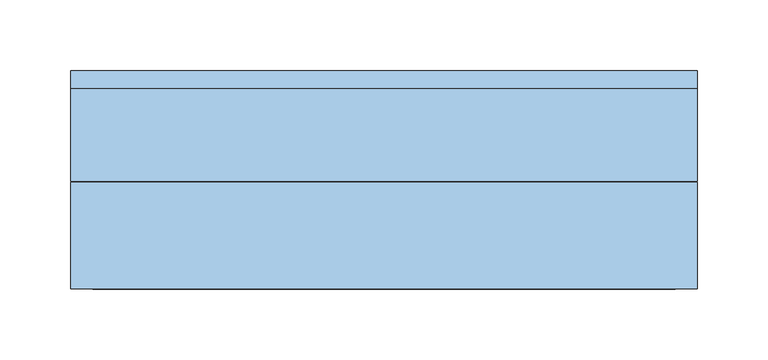
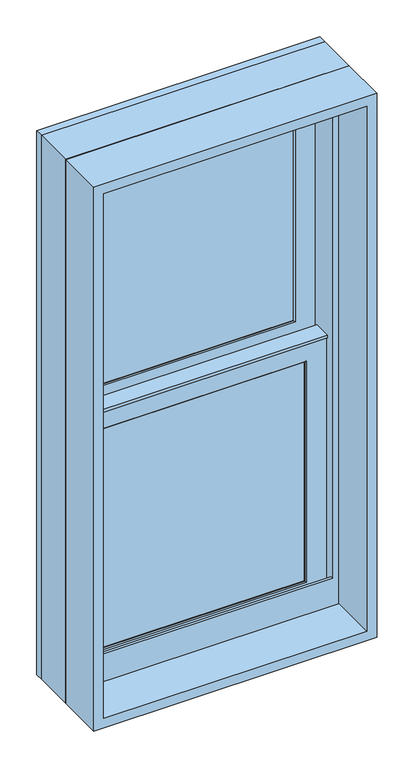
"""IFC4 building model written with IfcOpenShell, lengths in millimetres: window geometry, Window-Double_Hung-Marvin-Essential : ESDH1630."""

from ifc_helpers import new_model, si_unit, frame, origin, place, context, project, spatial, polyline, outline, extrude, faceted_brep, source, transform, mapped, element, save


def window_dba2cc00(model_context):
    return source(origin(), model_context, "Body", "SolidModel", [
        extrude(outline(polyline([(64.5583333, 20.6375), (64.5583333, 15.875), (45.5083333, 15.875), (45.5083333, 20.6375), (64.5583333, 20.6375)])), frame((0.0, 0.0, 1593.85), z_axis=(0.0, 0.0, 1.0), x_axis=(1.0, 0.0, 0.0)), (0.0, 0.0, 1.0), 374.65),
        extrude(outline(polyline([(-45.5083333, 20.6375), (-45.5083333, 15.875), (-64.5583333, 15.875), (-64.5583333, 20.6375), (-45.5083333, 20.6375)])), frame((0.0, 0.0, 1593.85), z_axis=(0.0, 0.0, 1.0), x_axis=(1.0, 0.0, 0.0)), (0.0, 0.0, 1.0), 374.65),
        extrude(outline(polyline([(165.1, 20.6375), (165.1, 15.875), (-165.1, 15.875), (-165.1, 20.6375), (165.1, 20.6375)])), frame((0.0, 0.0, 1771.65), z_axis=(0.0, 0.0, 1.0), x_axis=(1.0, 0.0, 0.0)), (0.0, 0.0, 1.0), 19.05),
        extrude(outline(polyline([(-64.5583333, 46.83125), (-64.5583333, 51.59375), (-45.5083333, 51.59375), (-45.5083333, 46.83125), (-64.5583333, 46.83125)])), frame((0.0, 0.0, 2006.6), z_axis=(0.0, 0.0, 1.0), x_axis=(1.0, 0.0, 0.0)), (0.0, 0.0, 1.0), 374.65),
        extrude(outline(polyline([(45.5083333, 46.83125), (45.5083333, 51.59375), (64.5583333, 51.59375), (64.5583333, 46.83125), (45.5083333, 46.83125)])), frame((0.0, 0.0, 2006.6), z_axis=(0.0, 0.0, 1.0), x_axis=(1.0, 0.0, 0.0)), (0.0, 0.0, 1.0), 374.65),
        extrude(outline(polyline([(-165.1, 46.83125), (-165.1, 51.59375), (165.1, 51.59375), (165.1, 46.83125), (-165.1, 46.83125)])), frame((0.0, 0.0, 2184.4), z_axis=(0.0, 0.0, 1.0), x_axis=(1.0, 0.0, 0.0)), (0.0, 0.0, 1.0), 19.05),
        extrude(outline(polyline([(64.5583333, 20.6375), (45.5083333, 20.6375), (45.5083333, 25.4), (64.5583333, 25.4), (64.5583333, 20.6375)])), frame((0.0, 0.0, 1593.85), z_axis=(0.0, 0.0, 1.0), x_axis=(1.0, 0.0, 0.0)), (0.0, 0.0, 1.0), 374.65),
        extrude(outline(polyline([(-45.5083333, 20.6375), (-64.5583333, 20.6375), (-64.5583333, 25.4), (-45.5083333, 25.4), (-45.5083333, 20.6375)])), frame((0.0, 0.0, 1593.85), z_axis=(0.0, 0.0, 1.0), x_axis=(1.0, 0.0, 0.0)), (0.0, 0.0, 1.0), 374.65),
        extrude(outline(polyline([(165.1, 20.6375), (-165.1, 20.6375), (-165.1, 25.4), (165.1, 25.4), (165.1, 20.6375)])), frame((0.0, 0.0, 1771.65), z_axis=(0.0, 0.0, 1.0), x_axis=(1.0, 0.0, 0.0)), (0.0, 0.0, 1.0), 19.05),
        extrude(outline(polyline([(-64.5583333, 56.35625), (-45.5083333, 56.35625), (-45.5083333, 51.59375), (-64.5583333, 51.59375), (-64.5583333, 56.35625)])), frame((0.0, 0.0, 2006.6), z_axis=(0.0, 0.0, 1.0), x_axis=(1.0, 0.0, 0.0)), (0.0, 0.0, 1.0), 374.65),
        extrude(outline(polyline([(45.5083333, 56.35625), (64.5583333, 56.35625), (64.5583333, 51.59375), (45.5083333, 51.59375), (45.5083333, 56.35625)])), frame((0.0, 0.0, 2006.6), z_axis=(0.0, 0.0, 1.0), x_axis=(1.0, 0.0, 0.0)), (0.0, 0.0, 1.0), 374.65),
        extrude(outline(polyline([(-165.1, 56.35625), (165.1, 56.35625), (165.1, 51.59375), (-165.1, 51.59375), (-165.1, 56.35625)])), frame((0.0, 0.0, 2184.4), z_axis=(0.0, 0.0, 1.0), x_axis=(1.0, 0.0, 0.0)), (0.0, 0.0, 1.0), 19.05),
        faceted_brep([(-192.0875, 5.6780605, 1998.5351748), (-192.0875, 5.6780605, 1993.9), (192.0875, 5.6780605, 1993.9), (192.0875, 5.6780605, 1998.5351748), (-192.0875, 34.8118605, 1998.5351748), (192.0875, 34.8118605, 1998.5351748), (192.0875, 34.8118605, 1993.9), (-192.0875, 34.8118605, 1993.9), (-192.0875, 30.1625, 1993.9), (-192.0875, 30.1625, 1566.8625), (-192.0875, 8.9241104, 1566.8625), (-192.0875, 8.9241104, 1993.9), (192.0875, 8.9241104, 1993.9), (192.0875, 30.1625, 1993.9), (192.0875, 8.9241104, 1566.8625), (192.0875, 30.1625, 1566.8625), (-176.2034752, 11.90625, 1979.6034752), (-176.2034752, 30.1625, 1979.6034752), (176.2034752, 30.1625, 1979.6034752), (176.2034752, 11.90625, 1979.6034752), (-159.54375, 10.4662439, 1962.94375), (-159.54375, 11.90625, 1962.94375), (159.54375, 11.90625, 1962.94375), (159.54375, 10.4662439, 1962.94375), (161.0858834, 8.9241104, 1964.4858834), (-161.0858834, 8.9241104, 1964.4858834), (176.2034752, 30.1625, 1582.7465248), (176.2034752, 11.90625, 1582.7465248), (159.54375, 11.90625, 1599.40625), (159.54375, 10.4662439, 1599.40625), (161.0858834, 8.9241104, 1597.8641166), (-176.2034752, 30.1625, 1582.7465248), (-176.2034752, 11.90625, 1582.7465248), (-159.54375, 11.90625, 1599.40625), (-159.54375, 10.4662439, 1599.40625), (-161.0858834, 8.9241104, 1597.8641166)], [[[0, 1, 2, 3]], [[4, 5, 6, 7]], [[1, 0, 4, 7, 8, 9, 10, 11]], [[2, 1, 11, 12]], [[7, 6, 13, 8]], [[3, 2, 12, 14, 15, 13, 6, 5]], [[0, 3, 5, 4]], [[16, 17, 18, 19]], [[20, 21, 22, 23]], [[20, 23, 24, 25]], [[19, 18, 26, 27]], [[23, 22, 28, 29]], [[24, 23, 29, 30]], [[27, 26, 31, 32]], [[29, 28, 33, 34]], [[30, 29, 34, 35]], [[15, 14, 10, 9]], [[15, 9, 8, 13], [18, 17, 31, 26]], [[17, 16, 32, 31]], [[16, 19, 27, 32], [22, 21, 33, 28]], [[21, 20, 34, 33]], [[20, 25, 35, 34]], [[10, 14, 12, 11], [25, 24, 30, 35]]]),
        extrude(outline(polyline([(38.5955581, 1979.6125), (33.5778968, 1979.6125), (33.5778968, 1981.2), (39.9405976, 1981.2), (39.9405976, 1979.6125), (61.515625, 1979.6125), (47.6307501, 1976.2975159), (38.5955581, 1976.2975159), (38.5955581, 1979.6125)])), frame((-192.0875, 0.0, 0.0), z_axis=(1.0, 0.0, 0.0), x_axis=(0.0, 1.0, 0.0)), (0.0, 0.0, 1.0), 384.175),
        faceted_brep([(222.25, 0.0, 1536.7), (222.25, 0.0, 2438.4), (-222.25, 0.0, 2438.4), (-222.25, 0.0, 1536.7), (196.05625, 0.0, 1597.81875), (-196.05625, 0.0, 1597.81875), (-196.05625, 0.0, 2412.20625), (196.05625, 0.0, 2412.20625), (196.05625, 3.96875, 1536.7), (-196.05625, 3.96875, 1536.7), (-196.05625, 3.96875, 1597.81875), (196.05625, 3.96875, 1597.81875), (-222.25, 65.6828125, 1536.7), (-196.05625, 65.6828125, 1536.7), (196.05625, 65.6828125, 1536.7), (222.25, 65.6828125, 1536.7), (-222.25, 65.6828125, 2438.4), (222.25, 65.6828125, 2438.4), (196.05625, 65.6828125, 2412.20625), (-196.05625, 65.6828125, 2412.20625)], [[[0, 1, 2, 3], [4, 5, 6, 7]], [[8, 9, 10, 11]], [[5, 4, 11, 10]], [[0, 3, 12, 13, 9, 8, 14, 15]], [[13, 12, 16, 17, 15, 14, 18, 19]], [[13, 19, 6, 5, 10, 9]], [[7, 6, 19, 18]], [[18, 14, 8, 11, 4, 7]], [[1, 0, 15, 17]], [[2, 1, 17, 16]], [[3, 2, 16, 12]]]),
        faceted_brep([(196.05625, 30.1625, 1987.55), (194.46875, 30.1625, 1987.55), (194.46875, 30.1625, 1561.0544613), (196.05625, 30.1625, 1561.0544613), (-194.46875, 30.1625, 1987.55), (-196.05625, 30.1625, 1987.55), (-196.05625, 30.1625, 1561.0544613), (-194.46875, 30.1625, 1561.0544613), (194.46875, 63.5, 1987.55), (196.05625, 63.5, 1987.55), (196.05625, 63.5, 1554.5743077), (194.46875, 63.5, 1554.5743077), (-196.05625, 63.5, 1987.55), (-194.46875, 63.5, 1987.55), (-194.46875, 63.5, 1554.5743077), (-196.05625, 63.5, 1554.5743077), (207.3108932, 3.96875, 1566.1460105), (207.3108932, 3.96875, 1536.7), (207.3108932, 65.6828125, 1536.7), (207.3108932, 65.6828125, 1554.150012), (-207.3108932, 3.96875, 1536.7), (-207.3108932, 3.96875, 1566.1460105), (-207.3108932, 65.6828125, 1554.150012), (-207.3108932, 65.6828125, 1536.7), (207.3108932, 78.58125, 1551.6428097), (-207.3108932, 78.58125, 1551.6428097), (-205.2971252, 68.2348864, 1553.6539391), (-187.33135, 68.2348864, 1553.6539391), (-187.33135, 65.6828125, 1554.150012), (187.33135, 65.6828125, 1554.150012), (187.33135, 68.2348864, 1553.6539391), (205.2971252, 68.2348864, 1553.6539391), (-222.25, 65.6828125, 1536.7), (-222.25, 78.5948249, 1536.7), (222.25, 78.5948249, 1536.7), (222.25, 65.6828125, 1536.7), (-222.25, 78.58125, 2438.4), (222.25, 78.58125, 2438.4), (207.3108932, 78.58125, 2423.4608932), (-207.3108932, 78.58125, 2423.4608932), (-222.25, 65.6828125, 2438.4), (-205.2971252, 68.2348864, 2421.4471252), (205.2971252, 68.2348864, 2421.4471252), (187.33135, 68.2348864, 2403.48135), (-187.33135, 68.2348864, 2403.48135), (-187.33135, 65.6828125, 2403.48135), (187.33135, 65.6828125, 2403.48135), (222.25, 65.6828125, 2438.4)], [[[0, 1, 2, 3]], [[4, 5, 6, 7]], [[8, 9, 10, 11]], [[12, 13, 14, 15]], [[1, 8, 11, 2]], [[9, 0, 3, 10]], [[1, 0, 9, 8]], [[5, 4, 13, 12]], [[5, 12, 15, 6]], [[13, 4, 7, 14]], [[16, 17, 18, 19]], [[20, 21, 22, 23]], [[24, 25, 26, 27, 28, 22, 21, 16, 19, 29, 30, 31], [3, 2, 11, 10], [7, 6, 15, 14]], [[17, 16, 21, 20]], [[17, 20, 23, 32, 33, 34, 35, 18]], [[34, 33, 36, 37], [25, 24, 38, 39]], [[33, 32, 40, 36]], [[39, 41, 26, 25]], [[41, 42, 31, 30, 43, 44, 27, 26]], [[44, 45, 28, 27]], [[40, 32, 23, 22, 28, 45, 46, 29, 19, 18, 35, 47]], [[36, 40, 47, 37]], [[39, 38, 42, 41]], [[44, 43, 46, 45]], [[34, 37, 47, 35]], [[42, 38, 24, 31]], [[46, 43, 30, 29]]]),
        extrude(outline(polyline([(172.24375, 11.90625), (-172.24375, 11.90625), (-172.24375, 15.08125), (172.24375, 15.08125), (172.24375, 11.90625)])), frame((0.0, 0.0, 1586.70625), z_axis=(0.0, 0.0, 1.0), x_axis=(1.0, 0.0, 0.0)), (0.0, 0.0, 1.0), 388.9375),
        extrude(outline(polyline([(172.24375, 42.8625), (-172.24375, 42.8625), (-172.24375, 46.0375), (172.24375, 46.0375), (172.24375, 42.8625)])), frame((0.0, 0.0, 1999.45625), z_axis=(0.0, 0.0, 1.0), x_axis=(1.0, 0.0, 0.0)), (0.0, 0.0, 1.0), 388.9375),
        faceted_brep([(-159.54375, 31.194477, 1962.94375), (-161.0858834, 32.7366104, 1964.4858834), (161.0858834, 32.7366104, 1964.4858834), (159.54375, 31.194477, 1962.94375), (-159.54375, 30.1625, 1962.94375), (159.54375, 30.1625, 1962.94375), (-192.0875, 32.7366104, 1995.4875), (-192.0875, 30.1625, 1995.4875), (192.0875, 30.1625, 1995.4875), (192.0875, 32.7366104, 1995.4875), (161.0858834, 32.7366104, 1597.8641166), (159.54375, 31.194477, 1599.40625), (159.54375, 30.1625, 1599.40625), (192.0875, 30.1625, 1566.8625), (192.0875, 32.7366104, 1566.8625), (-161.0858834, 32.7366104, 1597.8641166), (-159.54375, 31.194477, 1599.40625), (-159.54375, 30.1625, 1599.40625), (-192.0875, 30.1625, 1566.8625), (-192.0875, 32.7366104, 1566.8625)], [[[0, 1, 2, 3]], [[4, 0, 3, 5]], [[6, 7, 8, 9]], [[3, 2, 10, 11]], [[5, 3, 11, 12]], [[9, 8, 13, 14]], [[11, 10, 15, 16]], [[12, 11, 16, 17]], [[14, 13, 18, 19]], [[9, 14, 19, 6], [1, 15, 10, 2]], [[16, 15, 1, 0]], [[17, 16, 0, 4]], [[7, 18, 13, 8], [5, 12, 17, 4]], [[19, 18, 7, 6]]]),
        faceted_brep([(-176.2034752, 42.8625, 2392.3534752), (-176.2034752, 61.11875, 2392.3534752), (176.2034752, 61.11875, 2392.3534752), (176.2034752, 42.8625, 2392.3534752), (-159.54375, 41.4224939, 2375.69375), (-159.54375, 42.8625, 2375.69375), (159.54375, 42.8625, 2375.69375), (159.54375, 41.4224939, 2375.69375), (-161.0858834, 39.8803604, 2377.2358834), (161.0858834, 39.8803604, 2377.2358834), (-192.0875, 61.11875, 2408.2375), (-192.0875, 39.8803604, 2408.2375), (192.0875, 39.8803604, 2408.2375), (192.0875, 61.11875, 2408.2375), (176.2034752, 61.11875, 1995.4965248), (176.2034752, 42.8625, 1995.4965248), (159.54375, 42.8625, 2012.15625), (159.54375, 41.4224939, 2012.15625), (161.0858834, 39.8803604, 2010.6141166), (192.0875, 39.8803604, 1979.6125), (192.0875, 61.11875, 1979.6125), (-176.2034752, 61.11875, 1995.4965248), (-176.2034752, 42.8625, 1995.4965248), (-159.54375, 42.8625, 2012.15625), (-159.54375, 41.4224939, 2012.15625), (-161.0858834, 39.8803604, 2010.6141166), (-192.0875, 39.8803604, 1979.6125), (-192.0875, 61.11875, 1979.6125)], [[[0, 1, 2, 3]], [[4, 5, 6, 7]], [[8, 4, 7, 9]], [[10, 11, 12, 13]], [[3, 2, 14, 15]], [[7, 6, 16, 17]], [[9, 7, 17, 18]], [[13, 12, 19, 20]], [[15, 14, 21, 22]], [[17, 16, 23, 24]], [[18, 17, 24, 25]], [[20, 19, 26, 27]], [[13, 20, 27, 10], [1, 21, 14, 2]], [[22, 21, 1, 0]], [[3, 15, 22, 0], [5, 23, 16, 6]], [[24, 23, 5, 4]], [[25, 24, 4, 8]], [[11, 26, 19, 12], [9, 18, 25, 8]], [[27, 26, 11, 10]]]),
        faceted_brep([(-192.0875, 61.11875, 1979.6125), (-192.0875, 63.6928604, 1979.6125), (192.0875, 63.6928604, 1979.6125), (192.0875, 61.11875, 1979.6125), (-159.54375, 62.150727, 2012.15625), (-159.54375, 61.11875, 2012.15625), (159.54375, 61.11875, 2012.15625), (159.54375, 62.150727, 2012.15625), (-161.0858834, 63.6928604, 2010.6141166), (161.0858834, 63.6928604, 2010.6141166), (192.0875, 63.6928604, 2408.2375), (192.0875, 61.11875, 2408.2375), (159.54375, 61.11875, 2375.69375), (159.54375, 62.150727, 2375.69375), (161.0858834, 63.6928604, 2377.2358834), (-192.0875, 63.6928604, 2408.2375), (-192.0875, 61.11875, 2408.2375), (-159.54375, 61.11875, 2375.69375), (-159.54375, 62.150727, 2375.69375), (-161.0858834, 63.6928604, 2377.2358834)], [[[0, 1, 2, 3]], [[4, 5, 6, 7]], [[8, 4, 7, 9]], [[3, 2, 10, 11]], [[7, 6, 12, 13]], [[9, 7, 13, 14]], [[11, 10, 15, 16]], [[13, 12, 17, 18]], [[14, 13, 18, 19]], [[16, 15, 1, 0]], [[3, 11, 16, 0], [5, 17, 12, 6]], [[18, 17, 5, 4]], [[19, 18, 4, 8]], [[1, 15, 10, 2], [9, 14, 19, 8]]]),
        extrude(outline(polyline([(172.24375, 26.19375), (-172.24375, 26.19375), (-172.24375, 30.1625), (172.24375, 30.1625), (172.24375, 26.19375)])), frame((0.0, 0.0, 1586.70625), z_axis=(0.0, 0.0, 1.0), x_axis=(1.0, 0.0, 0.0)), (0.0, 0.0, 1.0), 388.9375),
        extrude(outline(polyline([(172.24375, 57.15), (-172.24375, 57.15), (-172.24375, 61.11875), (172.24375, 61.11875), (172.24375, 57.15)])), frame((0.0, 0.0, 1999.45625), z_axis=(0.0, 0.0, 1.0), x_axis=(1.0, 0.0, 0.0)), (0.0, 0.0, 1.0), 388.9375),
        extrude(outline(polyline([(2438.4, 222.25), (2438.4, -222.25), (1536.7, -222.25), (1536.7, 222.25), (2438.4, 222.25)]), holes=[polyline([(2422.525, 206.375), (1552.575, 206.375), (1552.575, -206.375), (2422.525, -206.375), (2422.525, 206.375)])]), frame((0.0, -76.2, 0.0), z_axis=(0.0, 1.0, 0.0), x_axis=(0.0, 0.0, 1.0)), (0.0, 0.0, 1.0), 75.40625),
    ])


if __name__ == "__main__":
    model = new_model("IFC4")
    model_context = context("Model", 3, world=origin())
    ifc_project = project(units=[si_unit("LENGTHUNIT", "METRE", prefix="MILLI")], contexts=[model_context])
    site = spatial("IfcSite", under=ifc_project)
    building = spatial("IfcBuilding", under=site)
    placement = place(None, origin())
    window_shape = window_dba2cc00(model_context)
    element("IfcWindow", 1, ObjectType="Window-Double_Hung-Marvin-Essential : ESDH1630", at=placement, inside=building, context=model_context, shape_type="MappedRepresentation", body=[
        mapped(window_shape, transform((0.0, 0.0, 0.0), x_axis=(1.0, 0.0, 0.0), y_axis=(0.0, 1.0, 0.0), z_axis=(0.0, 0.0, 1.0))),
    ])
    save(model, "model.ifc")

# Revit data of these elements
# Type "Window-Double_Hung-Marvin-Essential : ESDH1630"
#   Type Mark = "33"
#   Window Type = "Essential Double Hung"
#   Product data url = "https://bimobject.com/marvin-windows-and-doors/product/marvin-dhwau"
#   Product Guid = "c4a96547-874c-4385-91dc-a058adc19d98"
#   Frame = "All Ultrex"
#   Egress Window = "No"
#   URL = "www.marvin.com"
#   Model = "ESDH1630"
#   Manufacturer = "Marvin Windows and Doors"
#   Label Egress = ""
#   Glass Type = "IG Low E II with Argon"
#   Design Pressure = "DP50"
#   Description = "1836 DBHG"
#   Analytic Construction = "<None>"
#   Prairie Corner Width = 0' - 4"
#   Prairie Corner Height = 0' - 4"
#   Egress Width = 1' - 2 9/16"
#   Egress Height = 1' - 1 27/128"
#   Rough Width = 1' - 6"
#   Rough Height = 3' - 0"
#   Nominal Width = 1' - 6"
#   Nominal Height = 3' - 0"
#   Inset to Installation Flange [instance default] = 0' - 1"
#   Height = 2' - 11 1/2"
#   Egress Area = 1.336 SF
#   Default Head Height = 8' - 0"
#   Width = 1' - 5 1/2"
#   Daylight Area = 2.49723 SF
#   DLO Width = 1' - 0 9/16"
#   DLO Height = 1' - 2 5/16"
#   Muntins Top Sash = yes
#   Lites Wide Top Sash = 3
#   Lites Wide Bottom Sash = 3
#   Lites High Top Sash = 2
#   Lites High Bottom Sash = 2
#   Lite Cut Prairie 9 = no
#   Lite Cut HV Grid = yes
#   Muntins Bottom Sash = yes
#   Label Visibility = no
#   Jamb Extension Visibility = yes
#   Edition number = 1
#   Interior Material = Ultrex-Marvin-Stonewhite
#   Glazing Material = Glass-Marvin-IG Low E II with Argon
#   Cladding Material = Ultrex-Marvin-Pebblegray
#   Wall Closure = (empty or 0)
#   Assembly Code = ""
# Element 1 (IfcWindow, "Window-Double_Hung-Marvin-Essential : ESDH1630")
#   Materials on its faces: "Ultrex-Marvin-Pebblegray", "Ultrex-Marvin-Stonewhite", "Glass-Marvin-IG Low E II with Argon"
# Materials
#   "Ultrex-Marvin-Stonewhite": class "Paint", colour RGB 250 251 245, transparency 0
#   "Glass-Marvin-IG Low E II with Argon": class "Glass", colour RGB 0 128 192, transparency 0.85
#   "Ultrex-Marvin-Pebblegray": class "Paint", colour RGB 189 185 173, transparency 0
